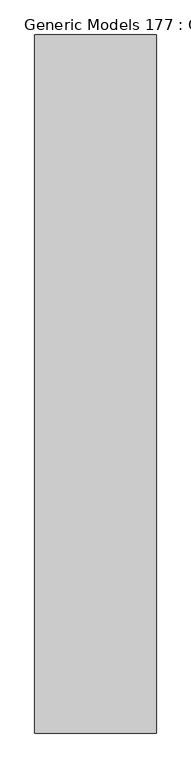
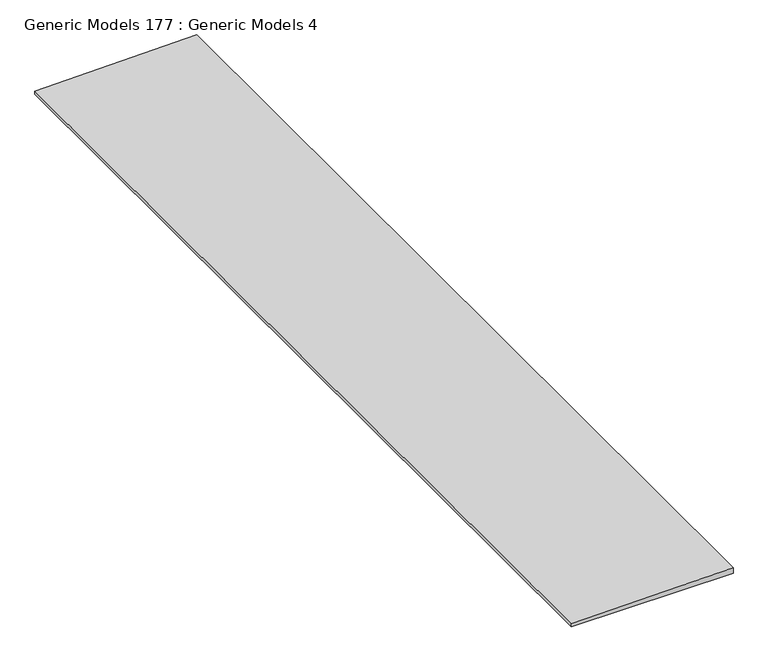
"""IFC4 building model written with IfcOpenShell, lengths in millimetres: proxy geometry, Generic Models 177 : Generic Models 4."""

from ifc_helpers import new_model, si_unit, frame, origin, place, context, project, spatial, polyline, outline, extrude, source, transform, mapped, element, save


def generic_models_177_generic_models_4_0921f90f(model_context):
    return source(origin(), model_context, "Body", "SweptSolid", [
        extrude(outline(polyline([(126663.196, -5311.9486296), (126711.4628099, -5311.9486296), (126688.596, -6621.9872911), (126663.196, -6621.9872911), (126663.196, -5311.9486296)])), frame((0.0, -464.1230338, 0.0), z_axis=(0.0, 1.0, 0.0), x_axis=(0.0, 0.0, 1.0)), (0.0, 0.0, 1.0), 7518.4),
    ])


if __name__ == "__main__":
    model = new_model("IFC4")
    model_context = context("Model", 3, world=origin())
    ifc_project = project(units=[si_unit("LENGTHUNIT", "METRE", prefix="MILLI")], contexts=[model_context])
    site = spatial("IfcSite", under=ifc_project)
    building = spatial("IfcBuilding", under=site)
    placement = place(None, origin())
    generic_models_177_generic_models_4_shape = generic_models_177_generic_models_4_0921f90f(model_context)
    element("IfcBuildingElementProxy", 1, Name="Generic Models 177 : Generic Models 4", ObjectType="Generic Models 177 : Generic Models 4", at=placement, inside=building, context=model_context, shape_type="MappedRepresentation", body=[
        mapped(generic_models_177_generic_models_4_shape, transform((0.0, 0.0, 0.0), x_axis=(1.0, 0.0, 0.0), y_axis=(0.0, 1.0, 0.0), z_axis=(0.0, 0.0, 1.0))),
    ])
    save(model, "model.ifc")

# Revit data of these elements
# Element 1 (IfcBuildingElementProxy, "Generic Models 177 : Generic Models 4")
#   Materials on its faces: "_TAPERED 2X BLOCKING (1% SLOPE)"
# Materials
#   "_TAPERED 2X BLOCKING (1% SLOPE)": class "Generic", colour RGB 177 130 114, transparency 0, Cost = 0
